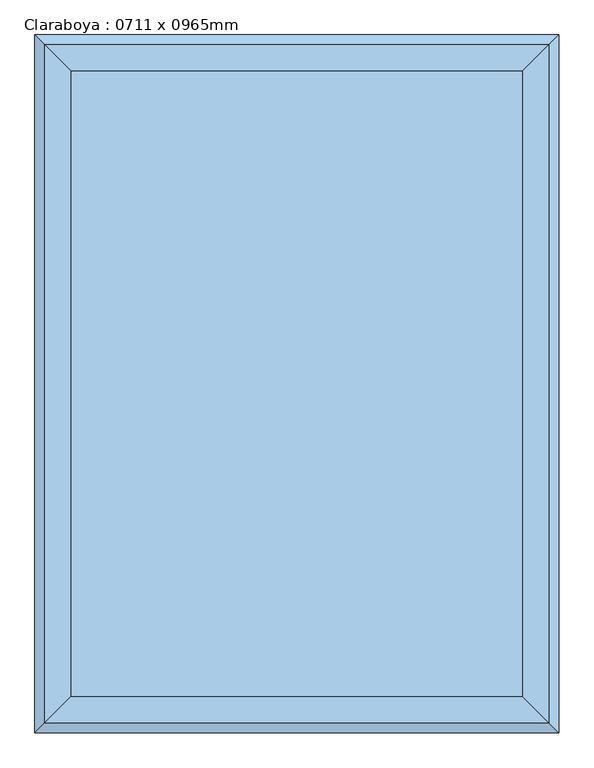
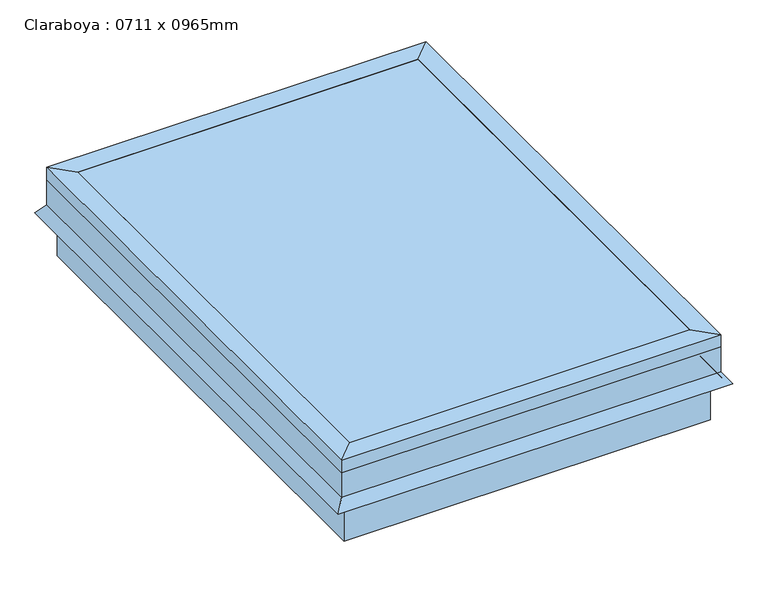
"""IFC4 building model written with IfcOpenShell, lengths in millimetres: window geometry, Claraboya : 0711 x 0965mm."""

from ifc_helpers import new_model, si_unit, frame, origin, place, context, project, spatial, polyline, outline, extrude, faceted_brep, source, transform, mapped, element, save


def claraboya_0711_x_0965mm_26b2130f(model_context):
    return source(origin(), model_context, "Body", "SolidModel", [
        faceted_brep([(254.440073, 370.1040988, 4001.2), (279.840073, 395.5040988, 4001.2), (279.840073, -569.4959012, 4001.2), (254.440073, -544.0959012, 4001.2), (254.440073, 370.1040988, 4026.6), (254.440073, -544.0959012, 4026.6), (292.540073, 408.2040988, 4026.6), (292.540073, -582.1959012, 4026.6), (292.540073, 408.2040988, 4001.2), (292.540073, -582.1959012, 4001.2), (292.540073, 408.2040988, 3950.4), (292.540073, -582.1959012, 3950.4), (307.1089145, 422.7729403, 3929.5935381), (307.1089145, -596.7647427, 3929.5935381), (301.907299, 417.5713248, 3925.9513277), (301.907299, -591.5631272, 3925.9513277), (286.190073, 401.8540988, 3948.3978527), (286.190073, -575.8459012, 3948.3978527), (286.190073, 401.8540988, 4001.2), (286.190073, -575.8459012, 4001.2), (-431.159927, -569.4959012, 4001.2), (-405.759927, -544.0959012, 4001.2), (-405.759927, -544.0959012, 4026.6), (-443.859927, -582.1959012, 4026.6), (-443.859927, -582.1959012, 4001.2), (-443.859927, -582.1959012, 3950.4), (-458.4287685, -596.7647427, 3929.5935381), (-453.227153, -591.5631272, 3925.9513277), (-437.509927, -575.8459012, 3948.3978527), (-437.509927, -575.8459012, 4001.2), (-431.159927, 395.5040988, 4001.2), (-405.759927, 370.1040988, 4001.2), (-405.759927, 370.1040988, 4026.6), (-443.859927, 408.2040988, 4026.6), (-443.859927, 408.2040988, 4001.2), (-443.859927, 408.2040988, 3950.4), (-458.4287685, 422.7729403, 3929.5935381), (-453.227153, 417.5713248, 3925.9513277), (-437.509927, 401.8540988, 3948.3978527), (-437.509927, 401.8540988, 4001.2)], [[[0, 1, 2, 3]], [[4, 0, 3, 5]], [[6, 4, 5, 7]], [[8, 6, 7, 9]], [[10, 8, 9, 11]], [[12, 10, 11, 13]], [[14, 12, 13, 15]], [[16, 14, 15, 17]], [[18, 16, 17, 19]], [[1, 18, 19, 2]], [[3, 2, 20, 21]], [[5, 3, 21, 22]], [[7, 5, 22, 23]], [[9, 7, 23, 24]], [[11, 9, 24, 25]], [[13, 11, 25, 26]], [[15, 13, 26, 27]], [[17, 15, 27, 28]], [[19, 17, 28, 29]], [[2, 19, 29, 20]], [[21, 20, 30, 31]], [[22, 21, 31, 32]], [[23, 22, 32, 33]], [[24, 23, 33, 34]], [[25, 24, 34, 35]], [[26, 25, 35, 36]], [[27, 26, 36, 37]], [[28, 27, 37, 38]], [[29, 28, 38, 39]], [[20, 29, 39, 30]], [[31, 30, 1, 0]], [[32, 31, 0, 4]], [[33, 32, 4, 6]], [[34, 33, 6, 8]], [[35, 34, 8, 10]], [[36, 35, 10, 12]], [[37, 36, 12, 14]], [[38, 37, 14, 16]], [[39, 38, 16, 18]], [[30, 39, 18, 1]]]),
        faceted_brep([(279.840073, -569.4959012, 4001.2), (279.840073, -569.4959012, 3848.8), (279.840073, 395.5040988, 3848.8), (279.840073, 395.5040988, 4001.2), (254.440073, -544.0959012, 4001.2), (254.440073, 370.1040988, 4001.2), (254.440073, -544.0959012, 3975.8), (254.440073, 370.1040988, 3975.8), (235.390073, -525.0459012, 3975.8), (235.390073, 351.0540988, 3975.8), (235.390073, -525.0459012, 3848.8), (235.390073, 351.0540988, 3848.8), (-431.159927, 395.5040988, 3848.8), (-431.159927, 395.5040988, 4001.2), (-405.759927, 370.1040988, 4001.2), (-405.759927, 370.1040988, 3975.8), (-386.709927, 351.0540988, 3975.8), (-386.709927, 351.0540988, 3848.8), (-431.159927, -569.4959012, 3848.8), (-431.159927, -569.4959012, 4001.2), (-405.759927, -544.0959012, 4001.2), (-405.759927, -544.0959012, 3975.8), (-386.709927, -525.0459012, 3975.8), (-386.709927, -525.0459012, 3848.8)], [[[0, 1, 2, 3]], [[4, 0, 3, 5]], [[6, 4, 5, 7]], [[8, 6, 7, 9]], [[10, 8, 9, 11]], [[1, 10, 11, 2]], [[3, 2, 12, 13]], [[5, 3, 13, 14]], [[7, 5, 14, 15]], [[9, 7, 15, 16]], [[11, 9, 16, 17]], [[2, 11, 17, 12]], [[13, 12, 18, 19]], [[14, 13, 19, 20]], [[15, 14, 20, 21]], [[16, 15, 21, 22]], [[17, 16, 22, 23]], [[12, 17, 23, 18]], [[19, 18, 1, 0]], [[20, 19, 0, 4]], [[21, 20, 4, 6]], [[22, 21, 6, 8]], [[23, 22, 8, 10]], [[18, 23, 10, 1]]]),
        extrude(outline(polyline([(254.440073, -544.0959012), (-405.759927, -544.0959012), (-405.759927, 370.1040988), (254.440073, 370.1040988), (254.440073, -544.0959012)])), frame((0.0, 0.0, 4020.25), z_axis=(0.0, 0.0, 1.0), x_axis=(1.0, 0.0, 0.0)), (0.0, 0.0, 1.0), 6.35),
    ])


if __name__ == "__main__":
    model = new_model("IFC4")
    model_context = context("Model", 3, world=origin())
    ifc_project = project(units=[si_unit("LENGTHUNIT", "METRE", prefix="MILLI")], contexts=[model_context])
    site = spatial("IfcSite", under=ifc_project)
    building = spatial("IfcBuilding", under=site)
    placement = place(None, origin())
    claraboya_0711_x_0965mm_shape = claraboya_0711_x_0965mm_26b2130f(model_context)
    element("IfcWindow", 1, ObjectType="Claraboya : 0711 x 0965mm", at=placement, inside=building, context=model_context, shape_type="MappedRepresentation", body=[
        mapped(claraboya_0711_x_0965mm_shape, transform((0.0, 0.0, 0.0), x_axis=(1.0, 0.0, 0.0), y_axis=(0.0, 1.0, 0.0), z_axis=(0.0, 0.0, 1.0))),
    ])
    save(model, "model.ifc")

# Revit data of these elements
# Type "Claraboya : 0711 x 0965mm"
#   Type Mark = "17"
#   Construction Type Id = "GSP4R"
#   Analytic Construction = "1/8 en cristalera simple Pilkington"
#   Visual Light Transmittance = 0.9
#   Solar Heat Gain Coefficient = 0.78
#   Heat Transfer Coefficient (U) = 3.6886 W/(m²·K)
#   Height = 0.965 m
#   Width = 0.711 m
#   Define Thermal Properties by = 1
#   Material de hoja = Metal - Bronce, Bruñido ligero
#   Material de hoja de cristal = Vidrio
#   Material de estructura = Metal - Bronce, Bruñido ligero
#   Type Comments = ""
# Element 1 (IfcWindow, "Claraboya : 0711 x 0965mm")
#   Materials on its faces: "Metal - Bronce, Bruñido ligero", "Vidrio"
# Materials
#   "Metal - Bronce, Bruñido ligero": class "Metal", colour RGB 113 80 70, transparency 0
#   "Vidrio": class "Vidrio", colour RGB 0 128 192, transparency 0.75, Description = "Vidrio de cal sodada", Cost = 0
